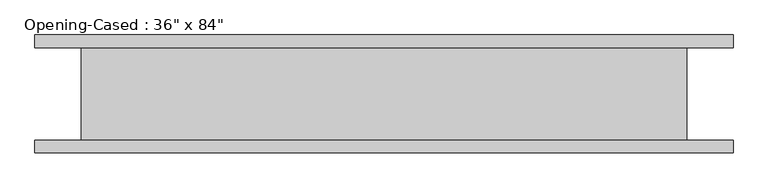
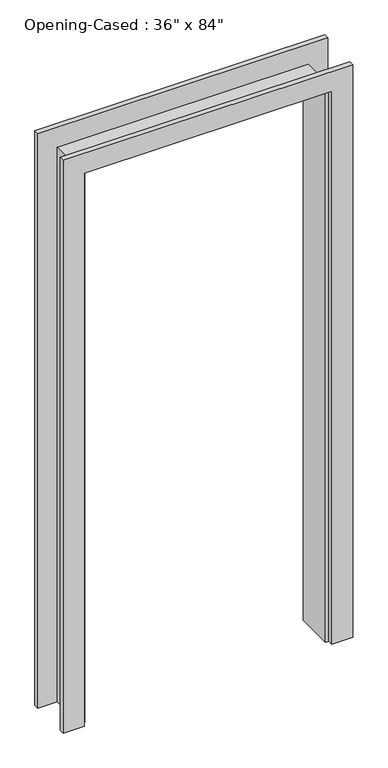
"""IFC4 building model written with IfcOpenShell, lengths in millimetres: proxy geometry."""

from ifc_helpers import new_model, si_unit, frame, origin, place, context, project, spatial, polyline, outline, extrude, faceted_brep, source, transform, mapped, element, save


def proxy_e62dbe84(model_context):
    return source(origin(), model_context, "Body", "SolidModel", [
        extrude(outline(polyline([(0.0, -459.0386567), (2127.25, -459.0386567), (2127.25, 442.6613433), (0.0, 442.6613433), (0.0, 518.8613433), (2203.45, 518.8613433), (2203.45, -535.2386567), (0.0, -535.2386567), (0.0, -459.0386567)])), frame((0.0, -88.9, 0.0), z_axis=(0.0, 1.0, 0.0), x_axis=(0.0, 0.0, 1.0)), (0.0, 0.0, 1.0), 19.05),
        extrude(outline(polyline([(0.0, 518.8613433), (2209.8, 518.8613433), (2209.8, -535.2386567), (0.0, -535.2386567), (0.0, -459.0386567), (2127.25, -459.0386567), (2127.25, 442.6613433), (0.0, 442.6613433), (0.0, 518.8613433)])), frame((0.0, 69.85, 0.0), z_axis=(0.0, 1.0, 0.0), x_axis=(0.0, 0.0, 1.0)), (0.0, 0.0, 1.0), 19.05),
        faceted_brep([(429.9613433, 69.85, 0.0), (449.0113433, 69.85, 0.0), (449.0113433, -69.85, 0.0), (429.9613433, -69.85, 0.0), (429.9613433, 69.85, 2114.55), (449.0113433, 69.85, 2133.6), (449.0113433, -69.85, 2133.6), (429.9613433, -69.85, 2114.55), (-446.3386567, 69.85, 2114.55), (-465.3886567, 69.85, 2133.6), (-465.3886567, -69.85, 2133.6), (-446.3386567, -69.85, 2114.55), (-446.3386567, 69.85, 0.0), (-446.3386567, -69.85, 0.0), (-465.3886567, -69.85, 0.0), (-465.3886567, 69.85, 0.0)], [[[0, 1, 2, 3]], [[1, 0, 4, 5]], [[2, 1, 5, 6]], [[3, 2, 6, 7]], [[0, 3, 7, 4]], [[5, 4, 8, 9]], [[6, 5, 9, 10]], [[7, 6, 10, 11]], [[4, 7, 11, 8]], [[12, 13, 14, 15]], [[9, 8, 12, 15]], [[10, 9, 15, 14]], [[11, 10, 14, 13]], [[8, 11, 13, 12]]]),
    ])


if __name__ == "__main__":
    model = new_model("IFC4")
    model_context = context("Model", 3, world=origin())
    ifc_project = project(units=[si_unit("LENGTHUNIT", "METRE", prefix="MILLI")], contexts=[model_context])
    site = spatial("IfcSite", under=ifc_project)
    building = spatial("IfcBuilding", under=site)
    placement = place(None, origin())
    proxy_shape = proxy_e62dbe84(model_context)
    element("IfcBuildingElementProxy", 1, Name="Opening-Cased : 36\" x 84\"", ObjectType="Opening-Cased : 36\" x 84\"", at=placement, inside=building, context=model_context, shape_type="MappedRepresentation", body=[
        mapped(proxy_shape, transform((0.0, 0.0, 0.0), x_axis=(1.0, 0.0, 0.0), y_axis=(0.0, 1.0, 0.0), z_axis=(0.0, 0.0, 1.0))),
    ])
    save(model, "model.ifc")

# Revit data of these elements
# Type "Opening-Cased : 36\" x 84\""
#   Height = 7' - 0"
#   Trim Thickness = 0' - 0 3/4"
#   Trim Width = 0' - 3"
#   Width = 3' - 0"
#   Frame Material = Trim - White
#   Assembly Code = ""
# Element 1 (IfcBuildingElementProxy, "Opening-Cased : 36\" x 84\"")
#   Materials on its faces: "Trim - White"
# Materials
#   "Trim - White": class "Paint", colour RGB 216 216 204, transparency 0
